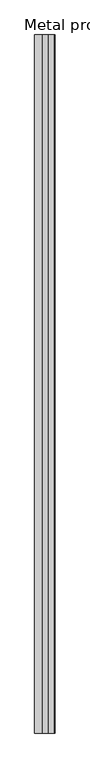
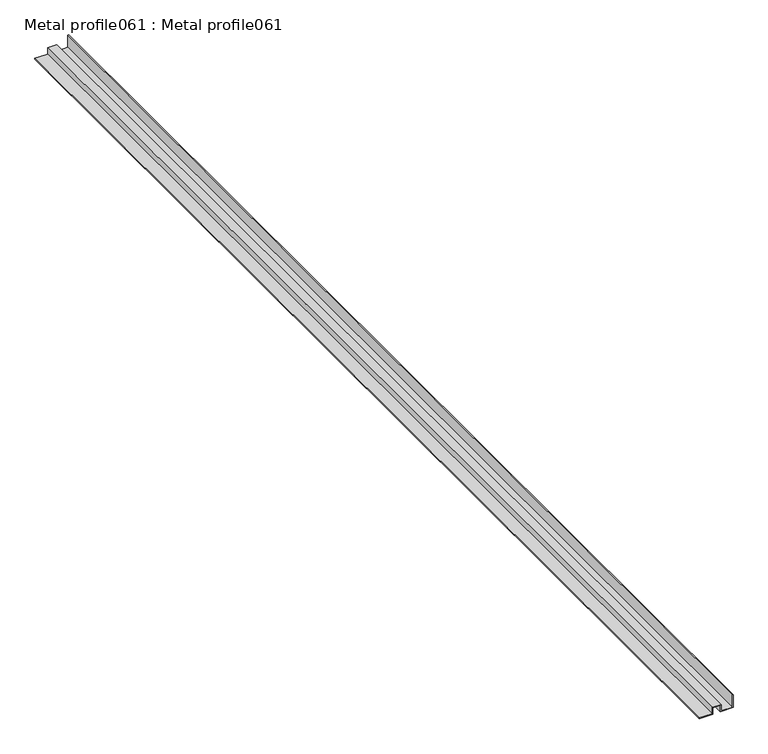
"""IFC4 building model written with IfcOpenShell, lengths in millimetres: proxy geometry, Metal profile061 : Metal profile061."""

from ifc_helpers import new_model, si_unit, frame, origin, place, context, project, spatial, polyline, outline, extrude, source, transform, mapped, element, save


def metal_profile061_metal_profile061_640eaa85(model_context):
    return source(origin(), model_context, "Body", "SweptSolid", [
        extrude(outline(polyline([(39543.8875708, -639.211476), (39567.6883323, -639.211476), (39567.6883323, -640.491476), (39545.1675708, -640.491476), (39545.1675708, -660.156476), (39556.5975708, -660.156476), (39556.5975708, -675.416476), (39545.1675708, -675.416476), (39545.1675708, -697.84966), (39543.8875708, -697.84966), (39543.8875708, -674.136476), (39555.3175708, -674.136476), (39555.3175708, -661.436476), (39543.8875708, -661.436476), (39543.8875708, -639.211476)])), frame((0.0, -1052.8906574, 0.0), z_axis=(0.0, 1.0, 0.0), x_axis=(0.0, 0.0, 1.0)), (0.0, 0.0, 1.0), 2000.0),
    ])


if __name__ == "__main__":
    model = new_model("IFC4")
    model_context = context("Model", 3, world=origin())
    ifc_project = project(units=[si_unit("LENGTHUNIT", "METRE", prefix="MILLI")], contexts=[model_context])
    site = spatial("IfcSite", under=ifc_project)
    building = spatial("IfcBuilding", under=site)
    placement = place(None, origin())
    metal_profile061_metal_profile061_shape = metal_profile061_metal_profile061_640eaa85(model_context)
    element("IfcBuildingElementProxy", 1, Name="Metal profile061 : Metal profile061", ObjectType="Metal profile061 : Metal profile061", at=placement, inside=building, context=model_context, shape_type="MappedRepresentation", body=[
        mapped(metal_profile061_metal_profile061_shape, transform((0.0, 0.0, 0.0), x_axis=(1.0, 0.0, 0.0), y_axis=(0.0, 1.0, 0.0), z_axis=(0.0, 0.0, 1.0))),
    ])
    save(model, "model.ifc")

# Revit data of these elements
# Type "Metal profile061 : Metal profile061"
#   NameOverride = "Metal profile061"
# Element 1 (IfcBuildingElementProxy, "Metal profile061 : Metal profile061")
#   Materials on its faces: "16 GA. COPPER SOFFIT DRIP SCREED"
# Materials
#   "16 GA. COPPER SOFFIT DRIP SCREED": class "Unassigned", colour RGB 255 217 0, transparency 0
